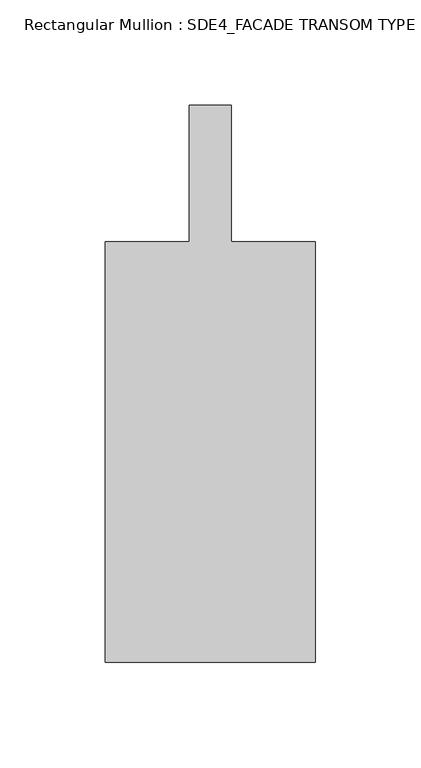
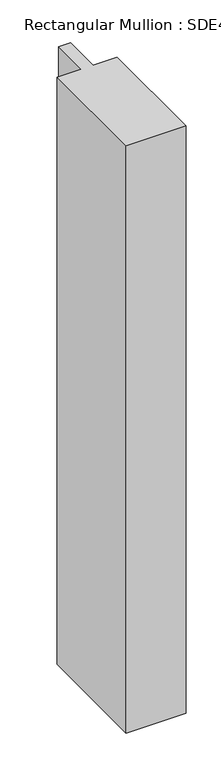
"""IFC4 building model written with IfcOpenShell, lengths in millimetres: member geometry, Rectangular Mullion : SDE4_FACADE TRANSOM TYPE 2."""

import ifcopenshell
import ifcopenshell.guid

model = None  # the IFC model being written
_history = None  # IfcOwnerHistory: only IFC2X3 demands one
_inside = {}  # id of a spatial element -> (the spatial element, [elements in it])
_under = {}  # id of a project, library or spatial element -> (it, [spatial elements below it])
_declared = {}  # id of a project -> (the project, [libraries it declares])
_typed = {}  # id of a type object -> (the type object, [elements of that type])
_made_of = {}  # id of a material, layer set ... -> (it, [elements and type objects made of it])


def new_model(schema):
    """Start an empty IFC model of exactly this schema.

    Asked for "IFC4X3", IfcOpenShell would pick the latest addendum, in which some entities
    have other attributes; the version numbers below select the first issue.
    IFC2X3 requires an IfcOwnerHistory on every rooted entity: one is made here for all.
    """
    global model, _history
    if schema == "IFC4X3":
        model = ifcopenshell.file(schema_version=(4, 3, 0, 0))
    else:
        model = ifcopenshell.file(schema=schema)
    _inside.clear()
    _under.clear()
    _declared.clear()
    _typed.clear()
    _made_of.clear()
    _history = None
    if model.schema == "IFC2X3":
        org = make("IfcOrganization", Name="unknown")
        user = make(
            "IfcPersonAndOrganization",
            ThePerson=make("IfcPerson", FamilyName="unknown"),
            TheOrganization=org,
        )
        app = make(
            "IfcApplication",
            ApplicationDeveloper=org,
            Version="unknown",
            ApplicationFullName="unknown",
            ApplicationIdentifier="unknown",
        )
        _history = make(
            "IfcOwnerHistory",
            OwningUser=user,
            OwningApplication=app,
            ChangeAction="ADDED",
            CreationDate=0,
        )
    return model


def make(cls, **values):
    """One entity of the class cls with the attributes given. An attribute that is None is left unset."""
    return model.create_entity(
        cls, **{name: value for name, value in values.items() if value is not None}
    )


def rooted(cls, **values):
    """An entity with a GlobalId (a new one), such as an element, a storey or a relation."""
    return make(cls, GlobalId=ifcopenshell.guid.new(), OwnerHistory=_history, **values)


def si_unit(unit_type, name, prefix=None):
    """IfcSIUnit, for example si_unit("LENGTHUNIT", "METRE", prefix="MILLI")."""
    return make("IfcSIUnit", UnitType=unit_type, Prefix=prefix, Name=name)


def assignment(units):
    """IfcUnitAssignment: the units of a project."""
    return None if units is None else make("IfcUnitAssignment", Units=units)


def point(xyz):
    """IfcCartesianPoint."""
    return None if xyz is None else make("IfcCartesianPoint", Coordinates=xyz)


def direction(xyz):
    """IfcDirection."""
    return None if xyz is None else make("IfcDirection", DirectionRatios=xyz)


def frame(location, z_axis=None, x_axis=None):
    """IfcAxis2Placement3D, a coordinate frame: its origin and axes. An axis left out is left unset."""
    return make(
        "IfcAxis2Placement3D",
        Location=point(location),
        Axis=direction(z_axis),
        RefDirection=direction(x_axis),
    )


def origin():
    """The frame at (0, 0, 0) with its axes left unset."""
    return frame((0.0, 0.0, 0.0))


def place(relative_to, where):
    """IfcLocalPlacement: puts the frame where relative to a parent placement (None: the world)."""
    return make(
        "IfcLocalPlacement", PlacementRelTo=relative_to, RelativePlacement=where
    )


def context(
    kind, dimensions, precision=None, world=None, true_north=None, identifier=None
):
    """IfcGeometricRepresentationContext, for example the 3D "Model" context."""
    return make(
        "IfcGeometricRepresentationContext",
        ContextIdentifier=identifier,
        ContextType=kind,
        CoordinateSpaceDimension=dimensions,
        Precision=precision,
        WorldCoordinateSystem=world,
        TrueNorth=true_north,
    )


def project(units=None, contexts=None):
    """IfcProject with its units and contexts."""
    return rooted(
        "IfcProject",
        Name="project",
        RepresentationContexts=contexts,
        UnitsInContext=assignment(units),
    )


def spatial(cls, under=None, at=None, **own):
    """A site, building, storey or space (cls), placed at a placement, below another one or the project."""
    s = rooted(cls, ObjectPlacement=at, **own)
    if under is not None:
        _under.setdefault(under.id(), (under, []))[1].append(s)
    return s


def polyline(points):
    """IfcPolyline through the points."""
    return make("IfcPolyline", Points=[point(p) for p in points])


def outline(outer, holes=None, kind="AREA"):
    """IfcArbitraryClosedProfileDef: a profile drawn as a closed curve; with holes, ...WithVoids."""
    if holes is None:
        return make("IfcArbitraryClosedProfileDef", ProfileType=kind, OuterCurve=outer)
    return make(
        "IfcArbitraryProfileDefWithVoids",
        ProfileType=kind,
        OuterCurve=outer,
        InnerCurves=holes,
    )


def extrude(swept, where, along, depth):
    """IfcExtrudedAreaSolid: the profile swept, set in the frame where, extruded along a direction by depth."""
    return make(
        "IfcExtrudedAreaSolid",
        SweptArea=swept,
        Position=where,
        ExtrudedDirection=direction(along),
        Depth=depth,
    )


def shape(context_of_items, identifier, shape_type, items):
    """IfcShapeRepresentation: the items that make up one representation, for example the "Body"."""
    return make(
        "IfcShapeRepresentation",
        ContextOfItems=context_of_items,
        RepresentationIdentifier=identifier,
        RepresentationType=shape_type,
        Items=items,
    )


def source(mapping_origin, context_of_items, identifier, shape_type, items):
    """IfcRepresentationMap: a shape defined once, which mapped items show again and again."""
    return make(
        "IfcRepresentationMap",
        MappingOrigin=mapping_origin,
        MappedRepresentation=shape(context_of_items, identifier, shape_type, items),
    )


def transform(
    local_origin,
    x_axis=None,
    y_axis=None,
    z_axis=None,
    scale=None,
    scale2=None,
    scale3=None,
    uniform=True,
):
    """IfcCartesianTransformationOperator3D, or its non-uniform kind. x_axis, y_axis, z_axis: its Axis1, 2, 3."""
    if uniform:
        return make(
            "IfcCartesianTransformationOperator3D",
            Axis1=direction(x_axis),
            Axis2=direction(y_axis),
            LocalOrigin=point(local_origin),
            Scale=scale,
            Axis3=direction(z_axis),
        )
    return make(
        "IfcCartesianTransformationOperator3DnonUniform",
        Axis1=direction(x_axis),
        Axis2=direction(y_axis),
        LocalOrigin=point(local_origin),
        Scale=scale,
        Axis3=direction(z_axis),
        Scale2=scale2,
        Scale3=scale3,
    )


def mapped(mapping_source, mapping_target):
    """IfcMappedItem: shows the shape of a source again, moved by a transform."""
    return make(
        "IfcMappedItem", MappingSource=mapping_source, MappingTarget=mapping_target
    )


def made_of(thing, what):
    """Note that an element or type object is made of a material, layer set ...; save() writes the relation."""
    if what is not None:
        _made_of.setdefault(what.id(), (what, []))[1].append(thing)
    return thing


def element(
    cls,
    number,
    at=None,
    inside=None,
    cuts=None,
    type_object=None,
    material=None,
    context=None,
    identifier="Body",
    shape_type=None,
    held_by="IfcProductDefinitionShape",
    body=None,
    shapes=None,
    **own,
):
    """One element of the class cls, such as IfcWall. Its Tag is "e" and its number.

    at: its placement. inside: the storey or other place that contains it. cuts: it is an
    opening in that element (IfcRelVoidsElement). A single representation is given by context,
    identifier, shape_type and body (its items); several are given by shapes. held_by: the class
    of the entity that holds the representations. save() writes the other relations.
    """
    e = rooted(cls, Tag="e%d" % number, ObjectPlacement=at, **own)
    if body is not None:
        shapes = [shape(context, identifier, shape_type, body)]
    if shapes is not None:
        e.Representation = make(held_by, Representations=shapes)
    if inside is not None:
        _inside.setdefault(inside.id(), (inside, []))[1].append(e)
    if cuts is not None:
        rooted(
            "IfcRelVoidsElement", RelatingBuildingElement=cuts, RelatedOpeningElement=e
        )
    if type_object is not None:
        _typed.setdefault(type_object.id(), (type_object, []))[1].append(e)
    return made_of(e, material)


def aggregate(whole, parts):
    """IfcRelAggregates: a whole, such as a stair, and the parts it consists of."""
    return rooted("IfcRelAggregates", RelatingObject=whole, RelatedObjects=parts)


def save(model, path):
    """Write the relations noted so far, then the file.

    IfcRelAggregates (storeys below a building ...), IfcRelContainedInSpatialStructure (elements
    in a storey), IfcRelDefinesByType, IfcRelAssociatesMaterial and IfcRelDeclares: one each for
    every whole, place, type object, material and project.
    """
    for whole, parts in _under.values():
        aggregate(whole, parts)
    for where, things in _inside.values():
        rooted(
            "IfcRelContainedInSpatialStructure",
            RelatedElements=things,
            RelatingStructure=where,
        )
    for kind, things in _typed.values():
        rooted("IfcRelDefinesByType", RelatedObjects=things, RelatingType=kind)
    for what, things in _made_of.values():
        rooted("IfcRelAssociatesMaterial", RelatedObjects=things, RelatingMaterial=what)
    for by, libraries in _declared.values():
        rooted("IfcRelDeclares", RelatingContext=by, RelatedDefinitions=libraries)
    model.write(path)


def rectangular_mullion_sde4_facade_transom_type_2_59b9a65e(model_context):
    return source(origin(), model_context, "Body", "SweptSolid", [
        extrude(outline(polyline([(50.0, -132.5), (-50.0, -132.5), (-50.0, 67.5), (-10.0, 67.5), (-10.0, 132.5), (10.0, 132.5), (10.0, 67.5), (50.0, 67.5), (50.0, -132.5)])), frame((0.0, 0.0, -1038.0000001), z_axis=(0.0, 0.0, 1.0), x_axis=(1.0, 0.0, 0.0)), (0.0, 0.0, 1.0), 1038.0000001),
    ])


if __name__ == "__main__":
    model = new_model("IFC4")
    model_context = context("Model", 3, world=origin())
    ifc_project = project(units=[si_unit("LENGTHUNIT", "METRE", prefix="MILLI")], contexts=[model_context])
    site = spatial("IfcSite", under=ifc_project)
    building = spatial("IfcBuilding", under=site)
    placement = place(None, origin())
    rectangular_mullion_sde4_facade_transom_type_2_shape = rectangular_mullion_sde4_facade_transom_type_2_59b9a65e(model_context)
    element("IfcMember", 1, ObjectType="Rectangular Mullion : SDE4_FACADE TRANSOM TYPE 2", at=placement, inside=building, context=model_context, shape_type="MappedRepresentation", body=[
        mapped(rectangular_mullion_sde4_facade_transom_type_2_shape, transform((0.0, 0.0, 0.0), x_axis=(1.0, 0.0, 0.0), y_axis=(0.0, 1.0, 0.0), z_axis=(0.0, 0.0, 1.0))),
    ])
    save(model, "model.ifc")

# Revit data of these elements
# Type "Rectangular Mullion : SDE4_FACADE TRANSOM TYPE 2"
#   built-in parameter 1007322 = 0.869423 (stored number, unit not read)
#   built-in parameter 1007321 = 0.164042 (stored number, unit not read)
#   built-in parameter 1007320 = 0.164042 (stored number, unit not read)
